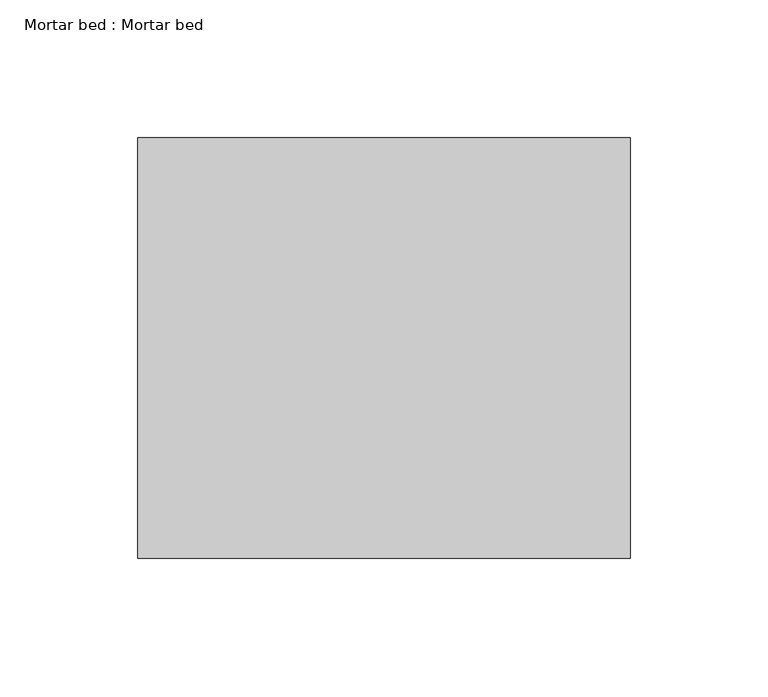
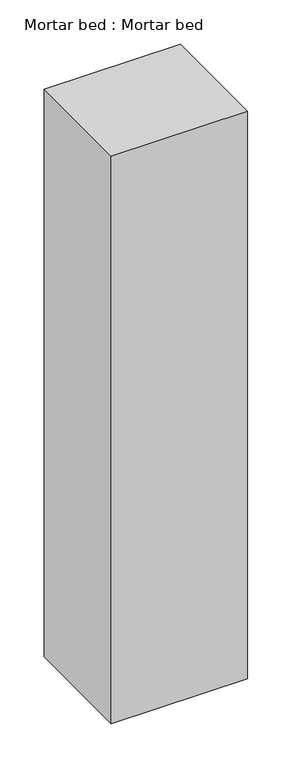
"""IFC4 building model written with IfcOpenShell, lengths in millimetres: proxy geometry, Mortar bed : Mortar bed."""

from ifc_helpers import new_model, si_unit, frame, origin, place, context, project, spatial, polyline, outline, extrude, source, transform, mapped, element, save


def mortar_bed_mortar_bed_deebc899(model_context):
    return source(origin(), model_context, "Body", "SweptSolid", [
        extrude(outline(polyline([(-10098.4737014, 9829.7531721), (-10276.8632813, 9829.7531721), (-10276.8632813, 9982.1531721), (-10098.4737014, 9982.1531721), (-10098.4737014, 9829.7531721)])), frame((0.0, 0.0, 32619.704006), z_axis=(0.0, 0.0, 1.0), x_axis=(1.0, 0.0, 0.0)), (0.0, 0.0, 1.0), 784.764744),
    ])


if __name__ == "__main__":
    model = new_model("IFC4")
    model_context = context("Model", 3, world=origin())
    ifc_project = project(units=[si_unit("LENGTHUNIT", "METRE", prefix="MILLI")], contexts=[model_context])
    site = spatial("IfcSite", under=ifc_project)
    building = spatial("IfcBuilding", under=site)
    placement = place(None, origin())
    mortar_bed_mortar_bed_shape = mortar_bed_mortar_bed_deebc899(model_context)
    element("IfcBuildingElementProxy", 1, Name="Mortar bed : Mortar bed", ObjectType="Mortar bed : Mortar bed", at=placement, inside=building, context=model_context, shape_type="MappedRepresentation", body=[
        mapped(mortar_bed_mortar_bed_shape, transform((0.0, 0.0, 0.0), x_axis=(1.0, 0.0, 0.0), y_axis=(0.0, 1.0, 0.0), z_axis=(0.0, 0.0, 1.0))),
    ])
    save(model, "model.ifc")

# Revit data of these elements
# Type "Mortar bed : Mortar bed"
#   NameOverride = "Mortar bed"
# Element 1 (IfcBuildingElementProxy, "Mortar bed : Mortar bed")
#   Materials on its faces: "MORTAR BED"
# Materials
#   "MORTAR BED": class "Unassigned", colour RGB 186 186 186, transparency 0, Cost = 0
